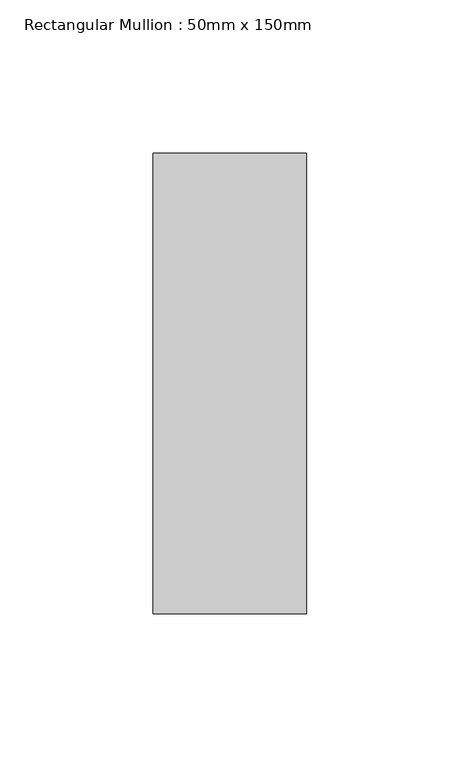
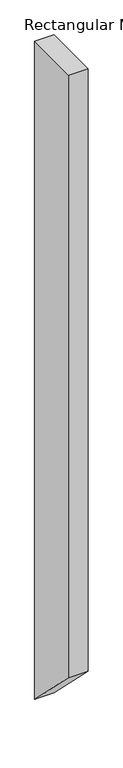
"""IFC4 building model written with IfcOpenShell, lengths in millimetres: member geometry, Rectangular Mullion : 50mm x 150mm."""

from ifc_helpers import new_model, si_unit, frame, origin, place, context, project, spatial, polyline, outline, extrude, source, transform, mapped, element, save


def rectangular_mullion_50mm_x_150mm_721863ff(model_context):
    return source(origin(), model_context, "Body", "SweptSolid", [
        extrude(outline(polyline([(-75.0, 0.0), (75.0, 0.0), (75.0, -1777.7272727), (-75.0, -1627.7272727), (-75.0, 0.0)])), frame((-25.0, 0.0, 0.0), z_axis=(1.0, 0.0, 0.0), x_axis=(0.0, 1.0, 0.0)), (0.0, 0.0, 1.0), 50.0),
    ])


if __name__ == "__main__":
    model = new_model("IFC4")
    model_context = context("Model", 3, world=origin())
    ifc_project = project(units=[si_unit("LENGTHUNIT", "METRE", prefix="MILLI")], contexts=[model_context])
    site = spatial("IfcSite", under=ifc_project)
    building = spatial("IfcBuilding", under=site)
    placement = place(None, origin())
    rectangular_mullion_50mm_x_150mm_shape = rectangular_mullion_50mm_x_150mm_721863ff(model_context)
    element("IfcMember", 1, ObjectType="Rectangular Mullion : 50mm x 150mm", at=placement, inside=building, context=model_context, shape_type="MappedRepresentation", body=[
        mapped(rectangular_mullion_50mm_x_150mm_shape, transform((0.0, 0.0, 0.0), x_axis=(1.0, 0.0, 0.0), y_axis=(0.0, 1.0, 0.0), z_axis=(0.0, 0.0, 1.0))),
    ])
    save(model, "model.ifc")

# Revit data of these elements
# Type "Rectangular Mullion : 50mm x 150mm"
#   built-in parameter 1007304 = 0.492126 (stored number, unit not read)
#   built-in parameter 1007301 = 0.082021 (stored number, unit not read)
#   built-in parameter 1007300 = 0.082021 (stored number, unit not read)
# Element 1 (IfcMember, "Rectangular Mullion : 50mm x 150mm")
#   Materials on its faces: "Aluminum"
# Materials
#   "Aluminum": class "Metal", colour RGB 244 244 244, transparency 0, Description = "Aluminum 6061", Cost = 0
